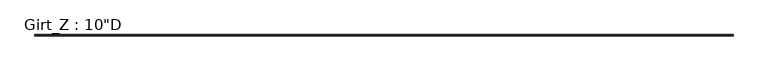
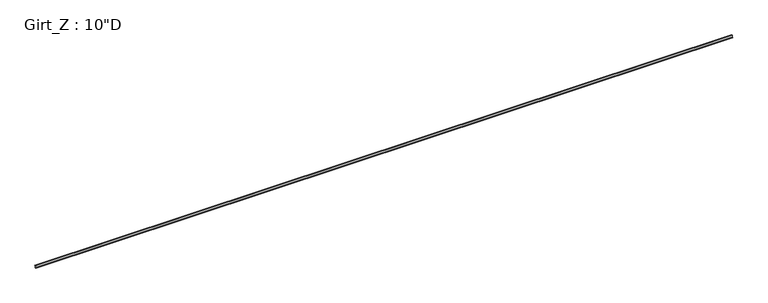
"""IFC4 building model written with IfcOpenShell, lengths in millimetres: beam geometry."""

from ifc_helpers import new_model, si_unit, point, frame, frame_2d, origin, place, context, project, spatial, polyline, circle_curve, trimmed, segment, composite_curve, outline, extrude, source, transform, mapped, element, save


def beam_b0892023(model_context):
    return source(origin(), model_context, "Body", "SweptSolid", [
        extrude(outline(composite_curve([segment(polyline([(77.9859375, 127.0), (90.2310415, 112.4068534), (88.1028742, 110.621109), (76.6904765, 124.221875), (3.3005807, 124.221875)]), True, "CONTINUOUS"), segment(trimmed(circle_curve(frame_2d((3.3741066, 122.2381931)), 1.9850441), [point((3.3005807, 124.221875))], [point((1.3890625, 122.2381931))], True, "CARTESIAN"), True, "CONTINUOUS"), segment(polyline([(1.3890625, 122.2381931), (1.3890625, -127.0), (-84.3359375, -127.0), (-96.5810415, -112.4068534), (-94.4528742, -110.621109), (-83.0404765, -124.221875), (-3.2694106, -124.221875)]), True, "CONTINUOUS"), segment(trimmed(circle_curve(frame_2d((-3.3748024, -122.2389339)), 1.9857399), [point((-3.2694106, -124.221875))], [point((-1.3890625, -122.2389339))], True, "CARTESIAN"), True, "CONTINUOUS"), segment(polyline([(-1.3890625, -122.2389339), (-1.3890625, 122.2375)]), True, "CONTINUOUS"), segment(trimmed(circle_curve(frame_2d((3.3734375, 122.2375)), 4.7625), [point((-1.3890625, 122.2375))], [point((3.3734375, 127.0))], False, "CARTESIAN"), True, "CONTINUOUS"), segment(polyline([(3.3734375, 127.0), (77.9859375, 127.0)]), True, "CONTINUOUS")], self_intersect=False)), frame((-44272.5320469, 0.0, 0.0), z_axis=(1.0, 0.0, 0.0), x_axis=(0.0, 1.0, 0.0)), (0.0, 0.0, 1.0), 88545.0640939),
    ])


if __name__ == "__main__":
    model = new_model("IFC4")
    model_context = context("Model", 3, world=origin())
    ifc_project = project(units=[si_unit("LENGTHUNIT", "METRE", prefix="MILLI")], contexts=[model_context])
    site = spatial("IfcSite", under=ifc_project)
    building = spatial("IfcBuilding", under=site)
    placement = place(None, origin())
    beam_shape = beam_b0892023(model_context)
    element("IfcBeam", 1, ObjectType="Girt_Z : 10\"D", at=placement, inside=building, context=model_context, shape_type="MappedRepresentation", body=[
        mapped(beam_shape, transform((0.0, 0.0, 0.0), x_axis=(1.0, 0.0, 0.0), y_axis=(0.0, 1.0, 0.0), z_axis=(0.0, 0.0, 1.0))),
    ])
    save(model, "model.ifc")

# Revit data of these elements
# Type "Girt_Z : 10\"D"
#   half leg = 0' - 1 11/16"
#   Web_Thickness = 0' - 0 7/64"
#   Length [instance default] = 10' - 0"
#   Leg_2 = 0' - 3 3/8"
#   Leg_1 = 0' - 3 1/8"
#   Height = 0' - 10"
#   Structural Material [instance default] = none
# Element 1 (IfcBeam, "Girt_Z : 10\"D")
#   Structural Material = STRUCTURAL STEEL - SEE STRUCT. DWGS
#   Materials on its faces: "STRUCTURAL STEEL - SEE STRUCT. DWGS"
# Materials
#   "STRUCTURAL STEEL - SEE STRUCT. DWGS": class "Metal", colour RGB 137 146 153, transparency 0, Description = "Steel, mill finish", Cost = 0
